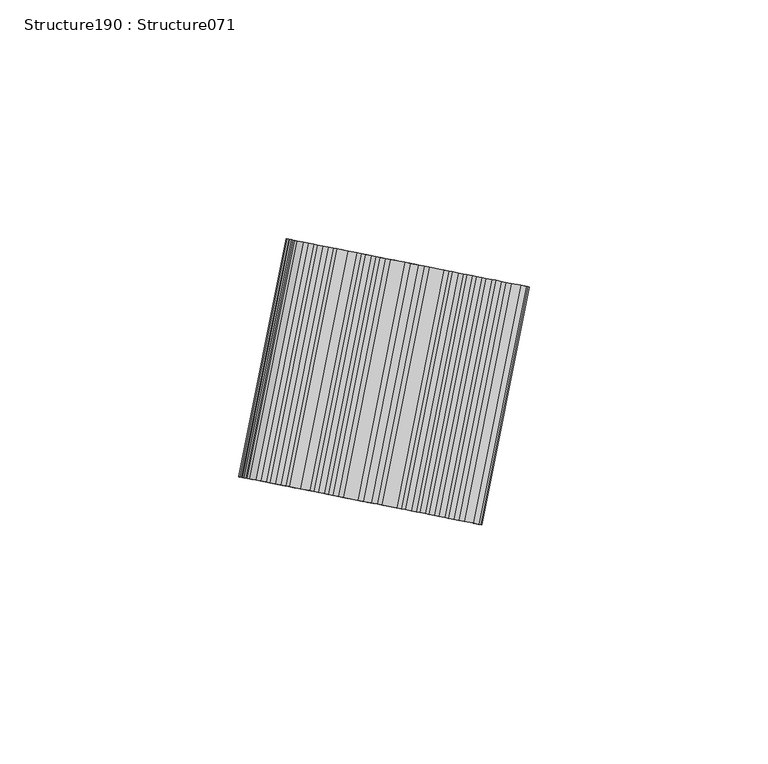
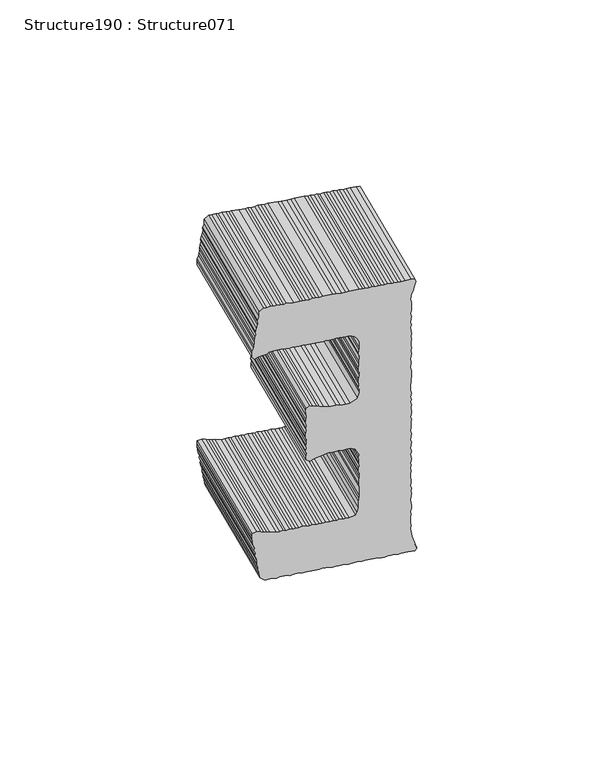
"""IFC4 building model written with IfcOpenShell, lengths in millimetres: proxy geometry, Structure190 : Structure071."""

from ifc_helpers import new_model, si_unit, frame, origin, place, context, project, spatial, polyline, outline, extrude, source, transform, mapped, element, save


def structure190_structure071_56f30129(model_context):
    return source(origin(), model_context, "Body", "SweptSolid", [
        extrude(outline(polyline([(1.4788121, 0.0), (2.2548681, -0.2742081), (3.0967006, -1.0995397), (4.8950919, -2.1683396), (5.4509723, -2.93455), (7.2984118, -4.3745158), (8.0716327, -4.6442584), (9.0174004, -5.5451874), (9.7579227, -6.2915538), (10.5762629, -6.9293998), (11.4550036, -7.2813885), (12.1121943, -8.1265642), (13.012562, -8.6591709), (15.4720729, -10.5762089), (16.0060457, -11.1615825), (17.6469357, -12.4405556), (18.728297, -12.9504748), (19.3698532, -13.6142896), (20.188474, -14.2523543), (21.0263777, -15.0746235), (21.7241249, -15.4493), (22.7273876, -16.0675206), (23.4404886, -16.6233392), (25.1267785, -18.2706345), (25.925836, -18.7242762), (26.6624293, -19.4675802), (29.8389702, -21.943499), (30.8229502, -22.3775152), (31.641571, -23.01558), (32.3024099, -23.8635992), (33.0978191, -24.3143973), (33.8341318, -25.0574825), (34.9452586, -25.7543631), (35.5805417, -26.4187019), (37.2175028, -27.6946127), (38.2233904, -28.3094658), (39.0456595, -28.9503742), (38.9190121, -30.1662599), (37.6061312, -30.7972524), (36.9441985, -31.4294483), (35.9171213, -32.1122281), (34.9685719, -32.6942587), (33.6440419, -33.9676065), (32.9042293, -34.7078235), (32.2887284, -35.7064392), (31.6250375, -36.3489941), (30.3456268, -37.9904454), (29.8097473, -38.8869089), (29.0699348, -39.6271258), (28.6390758, -40.6058975), (27.9187648, -41.5300382), (27.2570507, -42.1619536), (26.4330233, -43.0102162), (25.8175224, -44.0088319), (25.3601623, -44.8126601), (24.6177332, -45.5481309), (24.0844702, -46.4493406), (23.3190398, -47.0053779), (22.7829415, -47.9021219), (22.0650366, -48.8231756), (21.4024393, -49.4643274), (20.7639371, -50.2835095), (20.1484362, -51.2821252), (19.4062176, -52.0254292), (18.8690256, -52.9235765), (18.2064283, -53.5647283), (17.695073, -54.6467747), (16.8730225, -55.4843976), (16.2887341, -56.0250811), (15.858094, -57.0035721), (14.9310146, -57.7670007), (14.3938227, -58.665148), (13.7824695, -59.6665455), (13.0964417, -60.1207111), (12.4772222, -61.1240976), (12.0270805, -61.9186649), (11.09672, -62.6863031), (10.5608405, -63.5827666), (9.2838361, -65.2211308), (8.669858, -66.2258959), (7.9827365, -66.6814648), (7.3906661, -67.8670666), (6.8339727, -68.5812901), (6.0060162, -69.4264903), (5.473847, -70.3262968), (4.6327324, -70.9794348), (4.3560852, -71.7603566), (3.431412, -72.5206983), (2.918963, -73.6041479), (2.0741299, -74.2620567), (0.7947193, -75.903508), (0.33693, -76.6997837), (-0.3004785, -77.5175626), (-0.7541201, -78.3166201), (-2.1151208, -80.0627493), (-3.0384815, -80.8214071), (-4.1347731, -82.436865), (-4.9563944, -83.2820405), (-5.8678253, -84.8773737), (-6.689657, -85.714716), (-7.2251074, -86.6187321), (-8.0473766, -87.4566357), (-8.6856601, -88.2755372), (-9.0636176, -88.977494), (-9.8073592, -89.7146486), (-10.3428095, -90.6186647), (-11.9829815, -92.296973), (-12.2572225, -93.0748078), (-13.1009619, -93.7313134), (-13.7980529, -94.8346071), (-14.1736042, -95.5334768), (-15.1006835, -96.2969054), (-15.6109452, -97.3775487), (-17.3696152, -99.6338777), (-18.2927573, -100.3922548), (-19.2079067, -101.9923589), (-19.4100899, -103.3126793), (-20.0258095, -104.3115756), (-20.4599496, -105.2945568), (-20.7148377, -106.2489816), (-21.57793, -106.7288973), (-22.5885597, -106.1126037), (-24.1244911, -104.9154394), (-24.9610204, -104.0919858), (-25.7796413, -103.453921), (-26.7905515, -102.8374088), (-27.319221, -102.2539131), (-28.5058215, -101.6619665), (-29.0614213, -100.8959747), (-30.0684025, -100.2825249), (-30.6844028, -99.8023905), (-31.5209322, -98.9789368), (-32.2944337, -98.7089756), (-32.9552727, -97.8609564), (-34.1418732, -97.2690098), (-34.6795645, -96.6884069), (-35.5762137, -96.1510293), (-38.0357246, -94.2339914), (-38.7760364, -93.4954582), (-39.7220145, -92.586696), (-41.134237, -91.6573855), (-42.1361254, -91.0379804), (-44.5956363, -89.1209425), (-45.252827, -88.2757668), (-46.3381172, -87.7627854), (-47.0512183, -87.2069669), (-47.6110276, -86.4376941), (-48.6359172, -85.6388554), (-49.4324202, -85.1894606), (-50.0705384, -84.5206562), (-51.6061892, -83.3237106), (-53.61113, -82.0939179), (-54.0657001, -81.4066726), (-55.0454704, -80.9759375), (-55.9693306, -80.2558452), (-56.8148817, -79.4352845), (-57.5049813, -79.0588996), (-58.3505324, -78.2383389), (-59.1691533, -77.6002741), (-59.5520409, -75.9777631), (-58.4340605, -74.5434226), (-58.0446726, -73.1993911), (-57.3844814, -72.5613263), (-57.0052198, -71.8657996), (-56.6798187, -70.8052811), (-56.0798904, -69.6258041), (-55.4194805, -68.9874587), (-55.0671491, -68.109436), (-54.6277676, -67.1278333), (-54.0723866, -66.4152937), (-53.4573148, -65.4091254), (-53.0789282, -64.7147213), (-52.6702575, -63.5548942), (-52.2128972, -62.7510659), (-51.5746138, -61.9321644), (-50.3958036, -61.6983312), (-50.208394, -62.5026078), (-49.3624138, -63.330721), (-48.7020039, -64.1711876), (-47.9651918, -64.914211), (-47.7737912, -65.7220493), (-46.084282, -67.3646357), (-44.447321, -68.6405465), (-43.5681511, -69.0000879), (-42.6485006, -69.7168991), (-41.9838812, -70.5606468), (-41.00733, -70.9960909), (-40.294229, -71.5519094), (-39.6296095, -72.3956572), (-38.5259114, -73.0939656), (-36.0664005, -75.0110035), (-35.1686577, -75.5469779), (-34.4513471, -76.1060775), (-33.685698, -77.0285717), (-32.8104572, -77.3850507), (-31.8646894, -78.2859797), (-31.3314264, -78.8635821), (-29.6902557, -80.142774), (-28.7894589, -80.6829333), (-27.9480555, -81.5007123), (-26.2173558, -82.0295278), (-25.0431844, -81.784861), (-23.7331556, -81.1656307), (-22.2960333, -79.3218394), (-21.9167718, -78.6263128), (-21.3014896, -77.6279777), (-20.3761519, -76.8586803), (-19.4377906, -75.445843), (-18.7207607, -74.5259119), (-18.1054785, -73.5275768), (-17.5426603, -72.8054954), (-16.7030687, -72.1462081), (-16.1463752, -71.4319845), (-15.6262787, -70.3468265), (-15.0708977, -69.6342868), (-14.2492763, -68.7891112), (-13.7120844, -67.8909639), (-12.8720553, -67.2311153), (-12.3892959, -66.6117474), (-11.706384, -64.6740854), (-12.8293732, -62.3208744), (-13.7725161, -61.4165778), (-15.2068566, -60.2985973), (-16.3962924, -59.7021851), (-18.0332535, -58.4262743), (-19.7084267, -57.6172762), (-20.9733363, -57.1257979), (-21.8480777, -56.769257), (-22.9294391, -56.2593379), (-24.0700369, -56.0262583), (-24.3270901, -54.6682954), (-23.9550385, -53.9739159), (-22.4692971, -52.4937379), (-21.7743936, -51.3932507), (-21.396436, -50.691294), (-20.5553216, -50.038156), (-19.8577932, -48.9343011), (-19.2772234, -48.3983885), (-18.7630244, -47.3126939), (-18.046432, -46.393324), (-17.1989741, -45.7320475), (-16.5606905, -44.913146), (-16.0994014, -44.11238), (-15.4427101, -43.4788055), (-14.9324484, -42.3981623), (-14.1632995, -41.8373542), (-13.62742, -40.9408908), (-12.9095151, -40.0198371), (-11.4055763, -40.1959648), (-11.0069783, -41.1720677), (-10.4502848, -41.9366562), (-9.5843489, -42.9319042), (-9.0052568, -43.8853814), (-7.7054161, -45.3929685), (-6.910007, -45.8437665), (-5.9671447, -46.7478445), (-5.4305472, -47.3298505), (-4.2439466, -47.9217971), (-3.6128731, -48.5828548), (-2.6850841, -49.3060095), (-0.9508846, -49.8303349), (1.4256702, -48.8874973), (1.7060277, -48.1099184), (2.6024581, -47.1687647), (3.2409603, -46.3495826), (3.9048701, -45.7067469), (4.2576305, -44.8362769), (4.8983202, -44.0142884), (5.8212517, -43.248078), (6.459754, -42.4288958), (6.8379219, -41.7347723), (8.035305, -40.1985603), (8.8558327, -39.3547879), (10.7735268, -36.8944351), (11.1516947, -36.2003116), (11.7671956, -35.201696), (13.1260088, -33.4583731), (13.6726794, -31.9044491), (13.7445103, -30.9765171), (12.5266971, -29.3636907), (11.6260488, -28.8308651), (11.1717593, -28.1438387), (9.9851588, -27.551892), (9.5305887, -26.8646468), (8.6328458, -26.3286723), (7.7923173, -25.5097709), (6.6017879, -24.9147618), (5.9448777, -24.069805), (5.0468542, -23.5336118), (4.4089463, -22.8726407), (3.3239367, -22.3598779), (2.7680563, -21.5936675), (1.9716238, -21.1366582), (0.9696651, -20.5248675), (0.1019959, -19.5156369), (-0.6944366, -19.0586276), (-1.429726, -18.3217536), (-2.3123955, -17.9667025), (-3.1758551, -16.960753), (-3.9532856, -16.6877293), (-4.6101956, -15.8427725), (-5.4288165, -15.2047078), (-7.3923481, -14.3396756), (-8.2894966, -13.8023598), (-9.1680186, -13.4500903), (-10.1226003, -13.1959823), (-11.3118173, -12.5992895), (-12.2781802, -11.5158399), (-11.4782478, -10.489547), (-10.8408393, -9.671768), (-10.1537179, -9.2161992), (-9.253507, -8.270774), (-8.3032159, -7.694612), (-7.8495743, -6.8955546), (-6.8773757, -6.5002294), (-6.3419253, -5.5962134), (-5.4185646, -4.8375555), (-4.5555341, -4.3571405), (-3.7569141, -3.3325314), (-2.9914838, -2.7764941), (-2.4326029, -2.0594642), (-1.483554, -1.4773716), (-0.5858111, -0.5345341), (0.0, 0.0), (1.4788121, 0.0)])), frame((-2520.2344803, 234968.6402681, 387.6985279), z_axis=(0.19466222296394126, 0.9808703374813295, 0.0), x_axis=(0.7736290680390037, -0.15353339618842732, -0.614756505732107)), (0.0, 0.0, 1.0), 50.8),
    ])


if __name__ == "__main__":
    model = new_model("IFC4")
    model_context = context("Model", 3, world=origin())
    ifc_project = project(units=[si_unit("LENGTHUNIT", "METRE", prefix="MILLI")], contexts=[model_context])
    site = spatial("IfcSite", under=ifc_project)
    building = spatial("IfcBuilding", under=site)
    placement = place(None, origin())
    structure190_structure071_shape = structure190_structure071_56f30129(model_context)
    element("IfcBuildingElementProxy", 1, Name="Structure190 : Structure071", ObjectType="Structure190 : Structure071", at=placement, inside=building, context=model_context, shape_type="MappedRepresentation", body=[
        mapped(structure190_structure071_shape, transform((0.0, 0.0, 0.0), x_axis=(1.0, 0.0, 0.0), y_axis=(0.0, 1.0, 0.0), z_axis=(0.0, 0.0, 1.0))),
    ])
    save(model, "model.ifc")

# Revit data of these elements
# Type "Structure190 : Structure071"
#   NameOverride = "Structure071"
# Element 1 (IfcBuildingElementProxy, "Structure190 : Structure071")
#   Materials on its faces: "BRUSHED ALUMINUM LETTERING"
# Materials
#   "BRUSHED ALUMINUM LETTERING": class "Unassigned", colour RGB 169 181 186, transparency 0, Cost = 0
